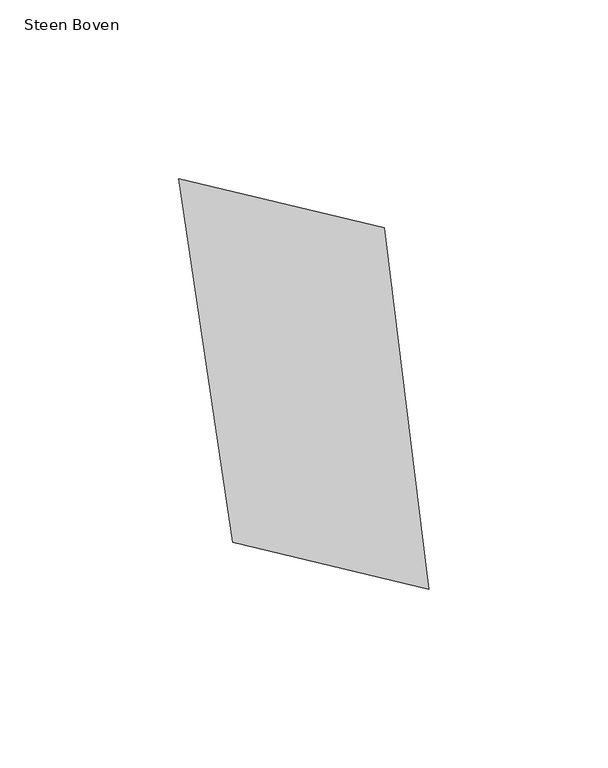
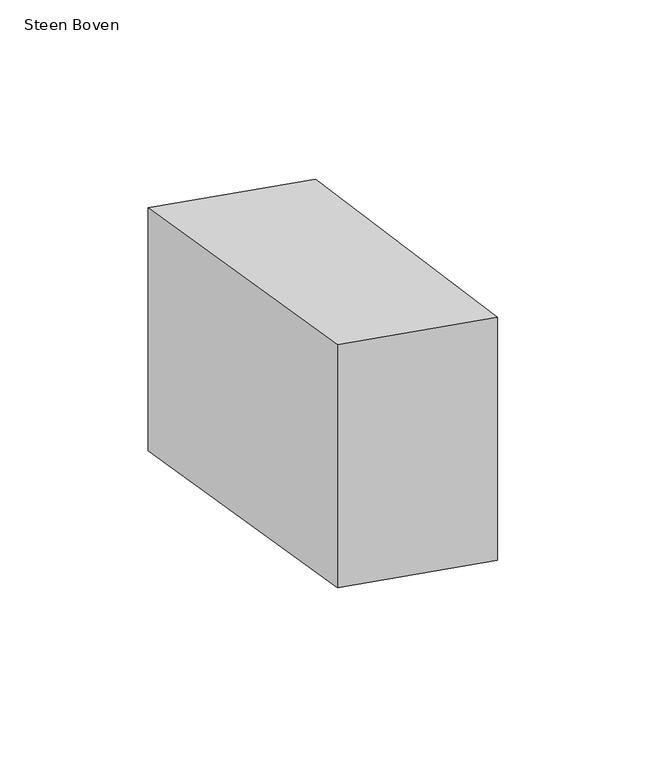
"""IFC4 building model written with IfcOpenShell, lengths in millimetres: proxy geometry, 00_GMA_steen_versie_4 : Steen Boven."""

from ifc_helpers import new_model, si_unit, origin, origin_with_axes, place, context, project, spatial, polyline, outline, extrude, source, transform, mapped, element, save


def steen_boven_21a2690e(model_context):
    return source(origin(), model_context, "Body", "SweptSolid", [
        extrude(outline(polyline([(94.1610985, 122.7087608), (106.6048076, 21.7602553), (51.8102366, 34.7745057), (36.8004137, 136.3719985), (94.1610985, 122.7087608)])), origin_with_axes(), (0.0, 0.0, 1.0), 100.0),
    ])


if __name__ == "__main__":
    model = new_model("IFC4")
    model_context = context("Model", 3, world=origin())
    ifc_project = project(units=[si_unit("LENGTHUNIT", "METRE", prefix="MILLI")], contexts=[model_context])
    site = spatial("IfcSite", under=ifc_project)
    building = spatial("IfcBuilding", under=site)
    placement = place(None, origin())
    steen_boven_shape = steen_boven_21a2690e(model_context)
    element("IfcBuildingElementProxy", 1, Name="00_GMA_steen_versie_4 : Steen Boven", ObjectType="00_GMA_steen_versie_4 : Steen Boven", at=placement, inside=building, context=model_context, shape_type="MappedRepresentation", body=[
        mapped(steen_boven_shape, transform((0.0, 0.0, 0.0), x_axis=(1.0, 0.0, 0.0), y_axis=(0.0, 1.0, 0.0), z_axis=(0.0, 0.0, 1.0))),
    ])
    save(model, "model.ifc")

# Revit data of these elements
# Type "00_GMA_steen_versie_4 : Steen Boven"
#   StootVoegHalfBoven [instance default] = 5 mm
#   StootVoegHalf [instance default] = 5 mm
#   StootVoegBreedteOnder = 10 mm
#   StootVoegBreedteBoven = 10 mm
#   Steendikte = 100 mm
#   LintVoegOnderHalf = 5 mm
#   LintVoegOnder = 10 mm
#   LintVoegBovenHalf = 0 mm
#   LintVoegBoven = 0 mm
#   materiaal = none
#   MateriaalVoeg = none
#   Default Elevation = 0
